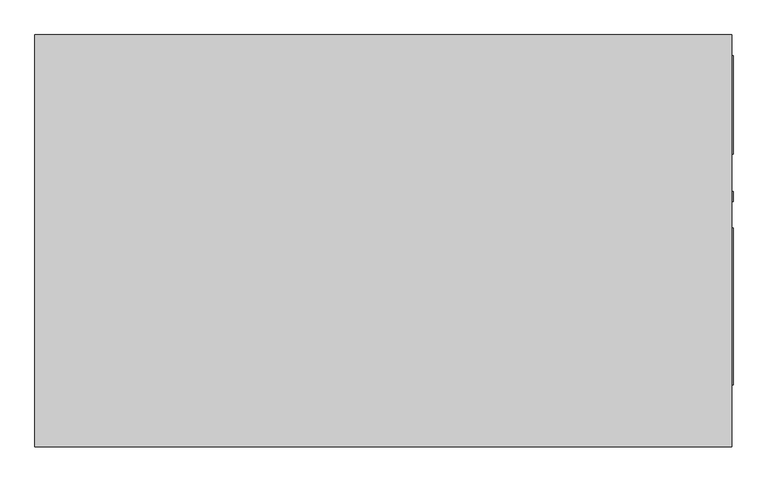
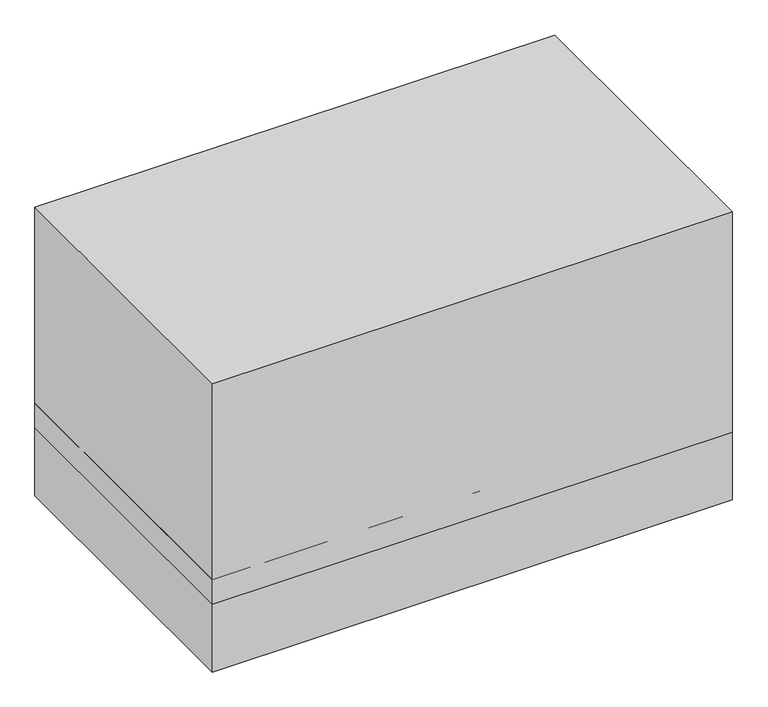
"""IFC4 building model written with IfcOpenShell, lengths in millimetres: proxy geometry, Carrier_48TC_Standard_Efficiency_Gas_Heat_Electric_Cooling_Packaged_Rooftop_Unit_3_to_15_nominal_tons : 5 ton 48TC**06."""

from ifc_helpers import new_model, si_unit, point, frame, frame_2d, origin, origin_with_axes, place, context, project, spatial, polyline, circle_curve, trimmed, segment, composite_curve, outline, extrude, source, transform, mapped, element, save
from ifc_brep_helpers import plane_surface, revolved_surface, advanced_brep


def mechanical_equipment_77e0781a(model_context):
    return source(origin(), model_context, "Body", "SolidModel", [
        extrude(outline(composite_curve([segment(trimmed(circle_curve(frame_2d((120.65, 438.15)), 13.2953125), [point((107.3546875, 438.15))], [point((133.9453125, 438.15))], False, "CARTESIAN"), True, "CONTINUOUS"), segment(trimmed(circle_curve(frame_2d((120.65, 438.15)), 13.2953125), [point((133.9453125, 438.15))], [point((107.3546875, 438.15))], False, "CARTESIAN"), True, "CONTINUOUS")], self_intersect=False)), frame((944.5625, 0.0, 0.0), z_axis=(1.0, 0.0, 0.0), x_axis=(0.0, 1.0, 0.0)), (0.0, 0.0, 1.0), 3.175),
        advanced_brep(
        [(944.5625, 558.8, 1108.075), (-944.5625, 558.8, 1108.075), (-944.5625, -558.8, 1108.075), (944.5625, -558.8, 1108.075), (944.5625, 558.8, 260.35), (944.5625, -558.8, 260.35), (-944.5625, -558.8, 260.35), (-944.5625, 558.8, 260.35), (858.8375, -400.05, 260.35), (858.8375, 0.0, 260.35), (550.8625, 0.0, 260.35), (550.8625, -400.05, 260.35), (858.8375, 463.55, 260.35), (207.9625, 463.55, 260.35), (207.9625, 187.325, 260.35), (858.8375, 187.325, 260.35), (284.7578125, -88.9, 260.35), (258.1671875, -88.9, 260.35), (-298.45, -247.65, 260.35), (-320.675, -247.65, 260.35), (-295.275, -149.225, 260.35), (-323.85, -149.225, 260.35), (-294.48125, -98.425, 260.35), (-324.64375, -98.425, 260.35), (858.8375, -400.05, 381.0), (550.8625, -400.05, 381.0), (550.8625, 0.0, 381.0), (858.8375, 0.0, 381.0), (858.8375, 463.55, 381.0), (858.8375, 187.325, 381.0), (207.9625, 187.325, 381.0), (207.9625, 463.55, 381.0), (284.7578125, -88.9, 415.925), (258.1671875, -88.9, 415.925), (-298.45, -247.65, 415.925), (-320.675, -247.65, 415.925), (-295.275, -149.225, 415.925), (-323.85, -149.225, 415.925), (-294.48125, -98.425, 415.925), (-324.64375, -98.425, 415.925)],
        [
            (0, 1),
            (1, 2),
            (2, 3),
            (3, 0),
            (4, 5),
            (5, 6),
            (6, 7),
            (7, 4),
            (8, 9),
            (9, 10),
            (10, 11),
            (11, 8),
            (12, 13),
            (13, 14),
            (14, 15),
            (15, 12),
            (16, 17, circle_curve(frame((271.4625, -88.9, 260.35), z_axis=(0.0, 0.0, 1.0), x_axis=(-1.0, 0.0, 0.0)), 13.2953125)),
            (17, 16, circle_curve(frame((271.4625, -88.9, 260.35), z_axis=(0.0, 0.0, 1.0), x_axis=(-1.0, 0.0, 0.0)), 13.2953125)),
            (18, 19, circle_curve(frame((-309.5625, -247.65, 260.35), z_axis=(0.0, 0.0, 1.0), x_axis=(-1.0, 0.0, 0.0)), 11.1125)),
            (19, 18, circle_curve(frame((-309.5625, -247.65, 260.35), z_axis=(0.0, 0.0, 1.0), x_axis=(-1.0, 0.0, 0.0)), 11.1125)),
            (20, 21, circle_curve(frame((-309.5625, -149.225, 260.35), z_axis=(0.0, 0.0, 1.0), x_axis=(-1.0, 0.0, 0.0)), 14.2875)),
            (21, 20, circle_curve(frame((-309.5625, -149.225, 260.35), z_axis=(0.0, 0.0, 1.0), x_axis=(-1.0, 0.0, 0.0)), 14.2875)),
            (22, 23, circle_curve(frame((-309.5625, -98.425, 260.35), z_axis=(0.0, 0.0, 1.0), x_axis=(-1.0, 0.0, 0.0)), 15.08125)),
            (23, 22, circle_curve(frame((-309.5625, -98.425, 260.35), z_axis=(0.0, 0.0, 1.0), x_axis=(-1.0, 0.0, 0.0)), 15.08125)),
            (0, 4),
            (7, 1),
            (6, 2),
            (5, 3),
            (24, 25),
            (25, 26),
            (26, 27),
            (27, 24),
            (27, 9),
            (8, 24),
            (26, 10),
            (25, 11),
            (28, 29),
            (29, 30),
            (30, 31),
            (31, 28),
            (31, 13),
            (12, 28),
            (30, 14),
            (29, 15),
            (32, 33, circle_curve(frame((271.4625, -88.9, 415.925), z_axis=(0.0, 0.0, -1.0), x_axis=(-1.0, 0.0, 0.0)), 13.2953125)),
            (33, 32, circle_curve(frame((271.4625, -88.9, 415.925), z_axis=(0.0, 0.0, -1.0), x_axis=(-1.0, 0.0, 0.0)), 13.2953125)),
            (33, 17),
            (16, 32),
            (34, 35, circle_curve(frame((-309.5625, -247.65, 415.925), z_axis=(0.0, 0.0, -1.0), x_axis=(-1.0, 0.0, 0.0)), 11.1125)),
            (35, 34, circle_curve(frame((-309.5625, -247.65, 415.925), z_axis=(0.0, 0.0, -1.0), x_axis=(-1.0, 0.0, 0.0)), 11.1125)),
            (35, 19),
            (18, 34),
            (36, 37, circle_curve(frame((-309.5625, -149.225, 415.925), z_axis=(0.0, 0.0, -1.0), x_axis=(-1.0, 0.0, 0.0)), 14.2875)),
            (37, 36, circle_curve(frame((-309.5625, -149.225, 415.925), z_axis=(0.0, 0.0, -1.0), x_axis=(-1.0, 0.0, 0.0)), 14.2875)),
            (37, 21),
            (20, 36),
            (38, 39, circle_curve(frame((-309.5625, -98.425, 415.925), z_axis=(0.0, 0.0, -1.0), x_axis=(-1.0, 0.0, 0.0)), 15.08125)),
            (39, 38, circle_curve(frame((-309.5625, -98.425, 415.925), z_axis=(0.0, 0.0, -1.0), x_axis=(-1.0, 0.0, 0.0)), 15.08125)),
            (39, 23),
            (22, 38),
        ],
        [
            plane_surface(frame((-944.5625, 558.8, 1108.075), z_axis=(0.0, 0.0, 1.0), x_axis=(-1.0, 0.0, 0.0))),
            plane_surface(frame((-944.5625, 558.8, 260.35), z_axis=(0.0, 0.0, -1.0), x_axis=(1.0, 0.0, 0.0))),
            plane_surface(frame((944.5625, 558.8, 1108.075), z_axis=(0.0, 1.0, 0.0), x_axis=(0.0, 0.0, -1.0))),
            plane_surface(frame((-944.5625, 558.8, 1108.075), z_axis=(-1.0, 0.0, 0.0), x_axis=(0.0, 0.0, -1.0))),
            plane_surface(frame((-944.5625, -558.8, 1108.075), z_axis=(0.0, -1.0, 0.0), x_axis=(0.0, 0.0, -1.0))),
            plane_surface(frame((944.5625, -558.8, 1108.075), z_axis=(1.0, 0.0, 0.0), x_axis=(0.0, 0.0, -1.0))),
            plane_surface(frame((858.8375, -400.05, 381.0), z_axis=(0.0, 0.0, -1.0), x_axis=(0.0, 1.0, 0.0))),
            plane_surface(frame((858.8375, -400.05, 381.0), z_axis=(-1.0, 0.0, 0.0), x_axis=(0.0, 0.0, -1.0))),
            plane_surface(frame((858.8375, 0.0, 381.0), z_axis=(0.0, -1.0, 0.0), x_axis=(0.0, 0.0, -1.0))),
            plane_surface(frame((550.8625, 0.0, 381.0), z_axis=(1.0, 0.0, 0.0), x_axis=(0.0, 0.0, -1.0))),
            plane_surface(frame((550.8625, -400.05, 381.0), z_axis=(0.0, 1.0, 0.0), x_axis=(0.0, 0.0, -1.0))),
            plane_surface(frame((207.9625, 463.55, 381.0), z_axis=(0.0, 0.0, -1.0), x_axis=(-1.0, 0.0, 0.0))),
            plane_surface(frame((858.8375, 463.55, 381.0), z_axis=(0.0, -1.0, 0.0), x_axis=(0.0, 0.0, -1.0))),
            plane_surface(frame((207.9625, 463.55, 381.0), z_axis=(1.0, 0.0, 0.0), x_axis=(0.0, 0.0, -1.0))),
            plane_surface(frame((207.9625, 187.325, 381.0), z_axis=(0.0, 1.0, 0.0), x_axis=(0.0, 0.0, -1.0))),
            plane_surface(frame((858.8375, 187.325, 381.0), z_axis=(-1.0, 0.0, 0.0), x_axis=(0.0, 0.0, -1.0))),
            plane_surface(frame((258.1671875, -88.9, 415.925), z_axis=(0.0, 0.0, -1.0), x_axis=(0.0, -1.0, 0.0))),
            revolved_surface(polyline([(258.16718749999995, -88.9, 415.925), (258.16718749999995, -88.9, 260.35)]), (271.4625, -88.9, 0.0), (0.0, 0.0, 1.0)),
            plane_surface(frame((-320.675, -247.65, 415.925), z_axis=(0.0, 0.0, -1.0), x_axis=(0.0, -1.0, 0.0))),
            revolved_surface(polyline([(-320.675, -247.65, 415.925), (-320.675, -247.65, 260.35)]), (-309.5625, -247.65, 0.0), (0.0, 0.0, 1.0)),
            plane_surface(frame((-323.85, -149.225, 415.925), z_axis=(0.0, 0.0, -1.0), x_axis=(0.0, -1.0, 0.0))),
            revolved_surface(polyline([(-323.85, -149.225, 415.925), (-323.85, -149.225, 260.35)]), (-309.5625, -149.225, 0.0), (0.0, 0.0, 1.0)),
            plane_surface(frame((-324.64375, -98.425, 415.925), z_axis=(0.0, 0.0, -1.0), x_axis=(0.0, -1.0, 0.0))),
            revolved_surface(polyline([(-324.64375, -98.425, 415.925), (-324.64375, -98.425, 260.35)]), (-309.5625, -98.425, 0.0), (0.0, 0.0, 1.0)),
        ],
        [
            (0, [[1, 2, 3, 4]]),
            (1, [[5, 6, 7, 8], [9, 10, 11, 12], [13, 14, 15, 16], [17, 18], [19, 20], [21, 22], [23, 24]]),
            (2, [[-1, 25, -8, 26]]),
            (3, [[-2, -26, -7, 27]]),
            (4, [[-3, -27, -6, 28]]),
            (5, [[-4, -28, -5, -25]]),
            (6, [[29, 30, 31, 32]]),
            (7, [[-32, 33, -9, 34]]),
            (8, [[-31, 35, -10, -33]]),
            (9, [[-30, 36, -11, -35]]),
            (10, [[-29, -34, -12, -36]]),
            (11, [[37, 38, 39, 40]]),
            (12, [[-40, 41, -13, 42]]),
            (13, [[-39, 43, -14, -41]]),
            (14, [[-38, 44, -15, -43]]),
            (15, [[-37, -42, -16, -44]]),
            (16, [[45, 46]]),
            (17, [[-46, 47, -17, 48]]),
            (17, [[-45, -48, -18, -47]]),
            (18, [[49, 50]]),
            (19, [[-50, 51, -19, 52]]),
            (19, [[-49, -52, -20, -51]]),
            (20, [[53, 54]]),
            (21, [[-54, 55, -21, 56]]),
            (21, [[-53, -56, -22, -55]]),
            (22, [[57, 58]]),
            (23, [[-58, 59, -23, 60]]),
            (23, [[-57, -60, -24, -59]]),
        ],
    ),
        extrude(outline(polyline([(944.5625, 558.8), (944.5625, -558.8), (-944.5625, -558.8), (-944.5625, 558.8), (944.5625, 558.8)]), holes=[polyline([(858.8375, 463.55), (207.9625, 463.55), (207.9625, 187.325), (858.8375, 187.325), (858.8375, 463.55)]), polyline([(858.8375, -400.05), (858.8375, 0.0), (550.8625, 0.0), (550.8625, -400.05), (858.8375, -400.05)]), composite_curve([segment(trimmed(circle_curve(frame_2d((271.4625, -88.9)), 13.2953125), [point((284.7578125, -88.9))], [point((258.1671875, -88.9))], True, "CARTESIAN"), True, "CONTINUOUS"), segment(trimmed(circle_curve(frame_2d((271.4625, -88.9)), 13.2953125), [point((258.1671875, -88.9))], [point((284.7578125, -88.9))], True, "CARTESIAN"), True, "CONTINUOUS")], self_intersect=False), composite_curve([segment(trimmed(circle_curve(frame_2d((-309.5625, -247.65)), 11.1125), [point((-298.45, -247.65))], [point((-320.675, -247.65))], True, "CARTESIAN"), True, "CONTINUOUS"), segment(trimmed(circle_curve(frame_2d((-309.5625, -247.65)), 11.1125), [point((-320.675, -247.65))], [point((-298.45, -247.65))], True, "CARTESIAN"), True, "CONTINUOUS")], self_intersect=False), composite_curve([segment(trimmed(circle_curve(frame_2d((-309.5625, -149.225)), 14.2875), [point((-295.275, -149.225))], [point((-323.85, -149.225))], True, "CARTESIAN"), True, "CONTINUOUS"), segment(trimmed(circle_curve(frame_2d((-309.5625, -149.225)), 14.2875), [point((-323.85, -149.225))], [point((-295.275, -149.225))], True, "CARTESIAN"), True, "CONTINUOUS")], self_intersect=False), composite_curve([segment(trimmed(circle_curve(frame_2d((-309.5625, -98.425)), 15.08125), [point((-294.48125, -98.425))], [point((-324.64375, -98.425))], True, "CARTESIAN"), True, "CONTINUOUS"), segment(trimmed(circle_curve(frame_2d((-309.5625, -98.425)), 15.08125), [point((-324.64375, -98.425))], [point((-294.48125, -98.425))], True, "CARTESIAN"), True, "CONTINUOUS")], self_intersect=False)]), origin_with_axes(), (0.0, 0.0, 1.0), 355.6),
        extrude(outline(polyline([(947.7375, 501.65), (947.7375, 234.95), (944.5625, 234.95), (944.5625, 501.65), (947.7375, 501.65)])), frame((0.0, 0.0, 412.75), z_axis=(0.0, 0.0, 1.0), x_axis=(1.0, 0.0, 0.0)), (0.0, 0.0, 1.0), 638.175),
        extrude(outline(polyline([(947.7375, 34.925), (947.7375, -390.525), (944.5625, -390.525), (944.5625, 34.925), (947.7375, 34.925)])), frame((0.0, 0.0, 415.925), z_axis=(0.0, 0.0, 1.0), x_axis=(1.0, 0.0, 0.0)), (0.0, 0.0, 1.0), 288.925),
    ])


if __name__ == "__main__":
    model = new_model("IFC4")
    model_context = context("Model", 3, world=origin())
    ifc_project = project(units=[si_unit("LENGTHUNIT", "METRE", prefix="MILLI")], contexts=[model_context])
    site = spatial("IfcSite", under=ifc_project)
    building = spatial("IfcBuilding", under=site)
    placement = place(None, origin())
    mechanical_equipment_shape = mechanical_equipment_77e0781a(model_context)
    element("IfcBuildingElementProxy", 1, Name="Carrier_48TC_Standard_Efficiency_Gas_Heat_Electric_Cooling_Packaged_Rooftop_Unit_3_to_15_nominal_tons : 5 ton 48TC**06", ObjectType="Carrier_48TC_Standard_Efficiency_Gas_Heat_Electric_Cooling_Packaged_Rooftop_Unit_3_to_15_nominal_tons : 5 ton 48TC**06", at=placement, inside=building, context=model_context, shape_type="MappedRepresentation", body=[
        mapped(mechanical_equipment_shape, transform((0.0, 0.0, 0.0), x_axis=(1.0, 0.0, 0.0), y_axis=(0.0, 1.0, 0.0), z_axis=(0.0, 0.0, 1.0))),
    ])
    save(model, "model.ifc")

# Revit data of these elements
# Type "Carrier_48TC_Standard_Efficiency_Gas_Heat_Electric_Cooling_Packaged_Rooftop_Unit_3_to_15_nominal_tons : 5 ton 48TC**06"
#   URL = "www.Carrier.com"
#   Model = "48TC"
#   Manufacturer = "Carrier"
#   Disclaimer = "Manufacturer reserves the right to change, at any time, specifications and designs without notice and without obligation.  Please verify critical parameters with local Carrier commercial sales office."
#   knockout thickness = 0' - 0 1/16"
#   Voltage = 0 V
#   Version = 1
#   TTBY3 = 1' - 0 1/4"
#   TTBY2 = 1' - 4 1/8"
#   TTBY1 = 1' - 6 1/8"
#   TTBX = 2' - 1"
#   TTBPowerR = 0' - 0 9/16"
#   TTBGasR = 0' - 0 19/32"
#   SSSZ = 0' - 6 1/8"
#   SSSY = 0' - 6 5/8"
#   SSSW = 1' - 4 3/4"
#   SSSH = 0' - 11 3/8"
#   SSRZ = 0' - 6"
#   SSRY = 0' - 2 1/4"
#   SSRW = 0' - 10 1/2"
#   SSRH = 2' - 1 1/8"
#   SEER = 13
#   Right clearance = 3' - 0"
#   PWRZ = 1' - 3 3/4"
#   PWRY = 0' - 4 5/8"
#   PWRR = 0' - 1 1/4"
#   ODF2X = 3' - 6"
#   ODF1Y = 1' - 2"
#   ODF1X = 1' - 2"
#   ODF1R = 1' - 1"
#   MOCP = 0 A
#   MCA = 0 A
#   Left clearance = 4' - 0"
#   IEER = 0
#   Front clearance = 4' - 0"
#   Fan Z = 3' - 7 5/8"
#   Width = 3' - 8"
#   Length = 6' - 2 3/8"
#   Height = 2' - 9 3/8"
#   EER = 10.75
#   DSSY = 0' - 6 1/4"
#   DSSX = 0' - 3 3/8"
#   DSSW = 1' - 0 1/8"
#   DSSH = 1' - 5 3/4"
#   DSRY = 0' - 3 3/4"
#   DSRX = 0' - 3 3/8"
#   DSRW = 2' - 1 5/8"
#   DSRH = 0' - 10 7/8"
#   DRNZ = 0' - 7"
#   DRNY = 2' - 2 3/4"
#   DRNR = 0' - 0 67/128"
#   Curb Z = 1' - 2"
#   CFM (nominal) = 0 CFM
#   Back clearance = 3' - 6"
#   Alt Condensate Drain = 0' - 0 67/128"
#   AccypwrR = 0' - 0 7/16"
#   ACY = 1' - 6 1/2"
#   ACX = 2' - 2 1/2"
#   Gas [instance default] = yes
#   Fan 2 on = no
#   Curb_1SLAB_2ROOFCURB_3SNOWCURB = 2
#   Fan 3 on = no
#   Unit material = American Sterling
#   Curb material = Curb paint
# Element 1 (IfcBuildingElementProxy, "Carrier_48TC_Standard_Efficiency_Gas_Heat_Electric_Cooling_Packaged_Rooftop_Unit_3_to_15_nominal_tons : 5 ton 48TC**06")
#   Materials on its faces: "American Sterling", "Curb paint", "Mech"
# Materials
#   "American Sterling": class "Miscellaneous", colour RGB 201 201 201, transparency 0, Cost = 0
#   "Curb paint": class "Miscellaneous", colour RGB 189 187 185, transparency 0
#   "Mech": class "Miscellaneous", colour RGB 235 237 235, transparency 0, Cost = 0
